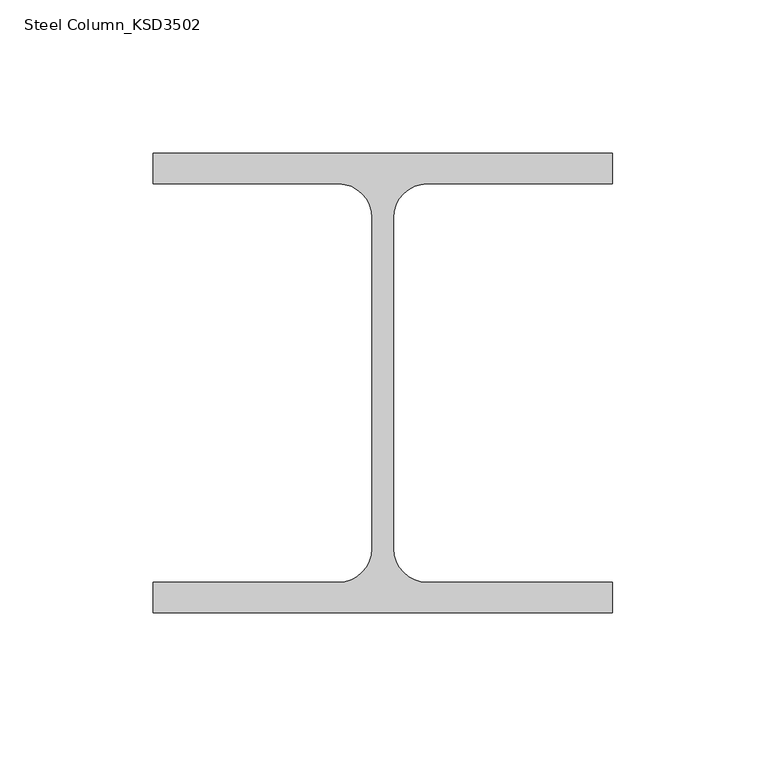
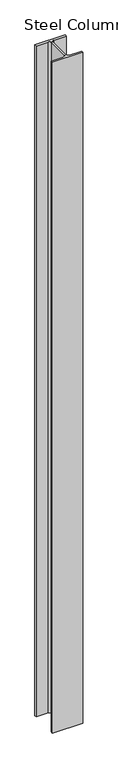
"""IFC4 building model written with IfcOpenShell, lengths in millimetres: column geometry, Steel Column_KSD3502 : H_SC_ASC_H-150×150x7x10."""

import ifcopenshell
import ifcopenshell.guid

model = None  # the IFC model being written
_history = None  # IfcOwnerHistory: only IFC2X3 demands one
_inside = {}  # id of a spatial element -> (the spatial element, [elements in it])
_under = {}  # id of a project, library or spatial element -> (it, [spatial elements below it])
_declared = {}  # id of a project -> (the project, [libraries it declares])
_typed = {}  # id of a type object -> (the type object, [elements of that type])
_made_of = {}  # id of a material, layer set ... -> (it, [elements and type objects made of it])


def new_model(schema):
    """Start an empty IFC model of exactly this schema.

    Asked for "IFC4X3", IfcOpenShell would pick the latest addendum, in which some entities
    have other attributes; the version numbers below select the first issue.
    IFC2X3 requires an IfcOwnerHistory on every rooted entity: one is made here for all.
    """
    global model, _history
    if schema == "IFC4X3":
        model = ifcopenshell.file(schema_version=(4, 3, 0, 0))
    else:
        model = ifcopenshell.file(schema=schema)
    _inside.clear()
    _under.clear()
    _declared.clear()
    _typed.clear()
    _made_of.clear()
    _history = None
    if model.schema == "IFC2X3":
        org = make("IfcOrganization", Name="unknown")
        user = make(
            "IfcPersonAndOrganization",
            ThePerson=make("IfcPerson", FamilyName="unknown"),
            TheOrganization=org,
        )
        app = make(
            "IfcApplication",
            ApplicationDeveloper=org,
            Version="unknown",
            ApplicationFullName="unknown",
            ApplicationIdentifier="unknown",
        )
        _history = make(
            "IfcOwnerHistory",
            OwningUser=user,
            OwningApplication=app,
            ChangeAction="ADDED",
            CreationDate=0,
        )
    return model


def make(cls, **values):
    """One entity of the class cls with the attributes given. An attribute that is None is left unset."""
    return model.create_entity(
        cls, **{name: value for name, value in values.items() if value is not None}
    )


def rooted(cls, **values):
    """An entity with a GlobalId (a new one), such as an element, a storey or a relation."""
    return make(cls, GlobalId=ifcopenshell.guid.new(), OwnerHistory=_history, **values)


def si_unit(unit_type, name, prefix=None):
    """IfcSIUnit, for example si_unit("LENGTHUNIT", "METRE", prefix="MILLI")."""
    return make("IfcSIUnit", UnitType=unit_type, Prefix=prefix, Name=name)


def assignment(units):
    """IfcUnitAssignment: the units of a project."""
    return None if units is None else make("IfcUnitAssignment", Units=units)


def point(xyz):
    """IfcCartesianPoint."""
    return None if xyz is None else make("IfcCartesianPoint", Coordinates=xyz)


def direction(xyz):
    """IfcDirection."""
    return None if xyz is None else make("IfcDirection", DirectionRatios=xyz)


def frame(location, z_axis=None, x_axis=None):
    """IfcAxis2Placement3D, a coordinate frame: its origin and axes. An axis left out is left unset."""
    return make(
        "IfcAxis2Placement3D",
        Location=point(location),
        Axis=direction(z_axis),
        RefDirection=direction(x_axis),
    )


def frame_2d(location, x_axis=None):
    """IfcAxis2Placement2D, a coordinate frame in the plane: its origin and x axis."""
    return make(
        "IfcAxis2Placement2D", Location=point(location), RefDirection=direction(x_axis)
    )


def origin():
    """The frame at (0, 0, 0) with its axes left unset."""
    return frame((0.0, 0.0, 0.0))


def place(relative_to, where):
    """IfcLocalPlacement: puts the frame where relative to a parent placement (None: the world)."""
    return make(
        "IfcLocalPlacement", PlacementRelTo=relative_to, RelativePlacement=where
    )


def context(
    kind, dimensions, precision=None, world=None, true_north=None, identifier=None
):
    """IfcGeometricRepresentationContext, for example the 3D "Model" context."""
    return make(
        "IfcGeometricRepresentationContext",
        ContextIdentifier=identifier,
        ContextType=kind,
        CoordinateSpaceDimension=dimensions,
        Precision=precision,
        WorldCoordinateSystem=world,
        TrueNorth=true_north,
    )


def project(units=None, contexts=None):
    """IfcProject with its units and contexts."""
    return rooted(
        "IfcProject",
        Name="project",
        RepresentationContexts=contexts,
        UnitsInContext=assignment(units),
    )


def spatial(cls, under=None, at=None, **own):
    """A site, building, storey or space (cls), placed at a placement, below another one or the project."""
    s = rooted(cls, ObjectPlacement=at, **own)
    if under is not None:
        _under.setdefault(under.id(), (under, []))[1].append(s)
    return s


def polyline(points):
    """IfcPolyline through the points."""
    return make("IfcPolyline", Points=[point(p) for p in points])


def circle_curve(where, radius):
    """IfcCircle in the frame where."""
    return make("IfcCircle", Position=where, Radius=radius)


def trimmed(basis, trim1, trim2, sense, master):
    """IfcTrimmedCurve: the piece of a basis curve between two trims."""
    return make(
        "IfcTrimmedCurve",
        BasisCurve=basis,
        Trim1=trim1,
        Trim2=trim2,
        SenseAgreement=sense,
        MasterRepresentation=master,
    )


def segment(curve, same_sense, transition):
    """IfcCompositeCurveSegment."""
    return make(
        "IfcCompositeCurveSegment",
        Transition=transition,
        SameSense=same_sense,
        ParentCurve=curve,
    )


def composite_curve(segments, self_intersect=None):
    """IfcCompositeCurve: segments joined end to end."""
    return make("IfcCompositeCurve", Segments=segments, SelfIntersect=self_intersect)


def outline(outer, holes=None, kind="AREA"):
    """IfcArbitraryClosedProfileDef: a profile drawn as a closed curve; with holes, ...WithVoids."""
    if holes is None:
        return make("IfcArbitraryClosedProfileDef", ProfileType=kind, OuterCurve=outer)
    return make(
        "IfcArbitraryProfileDefWithVoids",
        ProfileType=kind,
        OuterCurve=outer,
        InnerCurves=holes,
    )


def extrude(swept, where, along, depth):
    """IfcExtrudedAreaSolid: the profile swept, set in the frame where, extruded along a direction by depth."""
    return make(
        "IfcExtrudedAreaSolid",
        SweptArea=swept,
        Position=where,
        ExtrudedDirection=direction(along),
        Depth=depth,
    )


def shape(context_of_items, identifier, shape_type, items):
    """IfcShapeRepresentation: the items that make up one representation, for example the "Body"."""
    return make(
        "IfcShapeRepresentation",
        ContextOfItems=context_of_items,
        RepresentationIdentifier=identifier,
        RepresentationType=shape_type,
        Items=items,
    )


def source(mapping_origin, context_of_items, identifier, shape_type, items):
    """IfcRepresentationMap: a shape defined once, which mapped items show again and again."""
    return make(
        "IfcRepresentationMap",
        MappingOrigin=mapping_origin,
        MappedRepresentation=shape(context_of_items, identifier, shape_type, items),
    )


def transform(
    local_origin,
    x_axis=None,
    y_axis=None,
    z_axis=None,
    scale=None,
    scale2=None,
    scale3=None,
    uniform=True,
):
    """IfcCartesianTransformationOperator3D, or its non-uniform kind. x_axis, y_axis, z_axis: its Axis1, 2, 3."""
    if uniform:
        return make(
            "IfcCartesianTransformationOperator3D",
            Axis1=direction(x_axis),
            Axis2=direction(y_axis),
            LocalOrigin=point(local_origin),
            Scale=scale,
            Axis3=direction(z_axis),
        )
    return make(
        "IfcCartesianTransformationOperator3DnonUniform",
        Axis1=direction(x_axis),
        Axis2=direction(y_axis),
        LocalOrigin=point(local_origin),
        Scale=scale,
        Axis3=direction(z_axis),
        Scale2=scale2,
        Scale3=scale3,
    )


def mapped(mapping_source, mapping_target):
    """IfcMappedItem: shows the shape of a source again, moved by a transform."""
    return make(
        "IfcMappedItem", MappingSource=mapping_source, MappingTarget=mapping_target
    )


def made_of(thing, what):
    """Note that an element or type object is made of a material, layer set ...; save() writes the relation."""
    if what is not None:
        _made_of.setdefault(what.id(), (what, []))[1].append(thing)
    return thing


def element(
    cls,
    number,
    at=None,
    inside=None,
    cuts=None,
    type_object=None,
    material=None,
    context=None,
    identifier="Body",
    shape_type=None,
    held_by="IfcProductDefinitionShape",
    body=None,
    shapes=None,
    **own,
):
    """One element of the class cls, such as IfcWall. Its Tag is "e" and its number.

    at: its placement. inside: the storey or other place that contains it. cuts: it is an
    opening in that element (IfcRelVoidsElement). A single representation is given by context,
    identifier, shape_type and body (its items); several are given by shapes. held_by: the class
    of the entity that holds the representations. save() writes the other relations.
    """
    e = rooted(cls, Tag="e%d" % number, ObjectPlacement=at, **own)
    if body is not None:
        shapes = [shape(context, identifier, shape_type, body)]
    if shapes is not None:
        e.Representation = make(held_by, Representations=shapes)
    if inside is not None:
        _inside.setdefault(inside.id(), (inside, []))[1].append(e)
    if cuts is not None:
        rooted(
            "IfcRelVoidsElement", RelatingBuildingElement=cuts, RelatedOpeningElement=e
        )
    if type_object is not None:
        _typed.setdefault(type_object.id(), (type_object, []))[1].append(e)
    return made_of(e, material)


def aggregate(whole, parts):
    """IfcRelAggregates: a whole, such as a stair, and the parts it consists of."""
    return rooted("IfcRelAggregates", RelatingObject=whole, RelatedObjects=parts)


def save(model, path):
    """Write the relations noted so far, then the file.

    IfcRelAggregates (storeys below a building ...), IfcRelContainedInSpatialStructure (elements
    in a storey), IfcRelDefinesByType, IfcRelAssociatesMaterial and IfcRelDeclares: one each for
    every whole, place, type object, material and project.
    """
    for whole, parts in _under.values():
        aggregate(whole, parts)
    for where, things in _inside.values():
        rooted(
            "IfcRelContainedInSpatialStructure",
            RelatedElements=things,
            RelatingStructure=where,
        )
    for kind, things in _typed.values():
        rooted("IfcRelDefinesByType", RelatedObjects=things, RelatingType=kind)
    for what, things in _made_of.values():
        rooted("IfcRelAssociatesMaterial", RelatedObjects=things, RelatingMaterial=what)
    for by, libraries in _declared.values():
        rooted("IfcRelDeclares", RelatingContext=by, RelatedDefinitions=libraries)
    model.write(path)


def steel_column_ksd3502_e739ab66(model_context):
    return source(origin(), model_context, "Body", "SweptSolid", [
        extrude(outline(composite_curve([segment(polyline([(75.0, 75.0), (75.0, 65.0), (14.5, 65.0)]), True, "CONTINUOUS"), segment(trimmed(circle_curve(frame_2d((14.5, 54.0)), 11.0), [point((14.5, 65.0))], [point((3.5, 54.0))], True, "CARTESIAN"), True, "CONTINUOUS"), segment(polyline([(3.5, 54.0), (3.5, -54.0)]), True, "CONTINUOUS"), segment(trimmed(circle_curve(frame_2d((14.5, -54.0)), 11.0), [point((3.5, -54.0))], [point((14.5, -65.0))], True, "CARTESIAN"), True, "CONTINUOUS"), segment(polyline([(14.5, -65.0), (75.0, -65.0), (75.0, -75.0), (-75.0, -75.0), (-75.0, -65.0), (-14.5, -65.0)]), True, "CONTINUOUS"), segment(trimmed(circle_curve(frame_2d((-14.5, -54.0)), 11.0), [point((-14.5, -65.0))], [point((-3.5, -54.0))], True, "CARTESIAN"), True, "CONTINUOUS"), segment(polyline([(-3.5, -54.0), (-3.5, 54.0)]), True, "CONTINUOUS"), segment(trimmed(circle_curve(frame_2d((-14.5, 54.0)), 11.0), [point((-3.5, 54.0))], [point((-14.5, 65.0))], True, "CARTESIAN"), True, "CONTINUOUS"), segment(polyline([(-14.5, 65.0), (-75.0, 65.0), (-75.0, 75.0), (75.0, 75.0)]), True, "CONTINUOUS")], self_intersect=False)), frame((0.0, 0.0, 599.9720055), z_axis=(0.0, 0.0, 1.0), x_axis=(1.0, 0.0, 0.0)), (0.0, 0.0, 1.0), 3510.0),
    ])


if __name__ == "__main__":
    model = new_model("IFC4")
    model_context = context("Model", 3, world=origin())
    ifc_project = project(units=[si_unit("LENGTHUNIT", "METRE", prefix="MILLI")], contexts=[model_context])
    site = spatial("IfcSite", under=ifc_project)
    building = spatial("IfcBuilding", under=site)
    placement = place(None, origin())
    steel_column_ksd3502_shape = steel_column_ksd3502_e739ab66(model_context)
    element("IfcColumn", 1, ObjectType="Steel Column_KSD3502 : H_SC_ASC_H-150×150x7x10", at=placement, inside=building, context=model_context, shape_type="MappedRepresentation", body=[
        mapped(steel_column_ksd3502_shape, transform((0.0, 0.0, 0.0), x_axis=(1.0, 0.0, 0.0), y_axis=(0.0, 1.0, 0.0), z_axis=(0.0, 0.0, 1.0))),
    ])
    save(model, "model.ifc")

# Revit data of these elements
# Type "Steel Column_KSD3502 : H_SC_ASC_H-150×150x7x10"
#   Width = 15.0 cm
#   Web Thickness = 0.7 cm
#   Web Fillet = 1.1 cm
#   Warping Constant = 27562.5 cm⁶
#   Torsional Moment of Inertia = 11.6007 cm⁴
#   Section Area = 40.14 cm²
#   Plastic Modulus weak axis = 115.0 cm³
#   Plastic Modulus strong axis = 246.0 cm³
#   Perimeter = 1.27 m²/m
#   Nominal Weight = 31.50 kgf/m
#   Moment of Inertia weak axis = 563.00 cm⁴
#   Moment of Inertia strong axis = 1640.00 cm⁴
#   Height = 15.0 cm
#   Flange Thickness = 1.0 cm
#   Elastic Modulus weak axis = 75.1 cm³
#   Elastic Modulus strong axis = 219.0 cm³
#   Centroid Vertical = 7.5 cm
#   Centroid Horizontal = 7.5 cm
#   Bolt Spacing = 13.97 cm
#   Structural Material [instance default] = Steel, 45-345
#   Section Name Key = ""
#   Assembly Code = ""
# Element 1 (IfcColumn, "Steel Column_KSD3502 : H_SC_ASC_H-150×150x7x10")
#   Structural Material = A03AD029-00005_Anchor Bolt (Installation only)_M24
#   Materials on its faces: "A03AD029-00005_Anchor Bolt (Installation only)_M24"
# Materials
#   "Steel, 45-345": class "Metal", colour RGB 189 187 185, transparency 0, Description = "Steel 345 MPa", Cost = 0
#   "A03AD029-00005_Anchor Bolt (Installation only)_M24": class "Unassigned", colour RGB 84 83 81, transparency 0, Cost = 0
